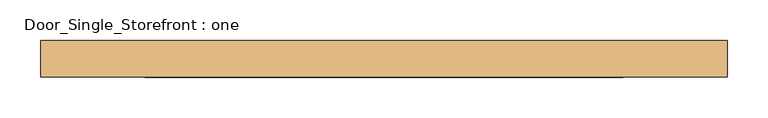
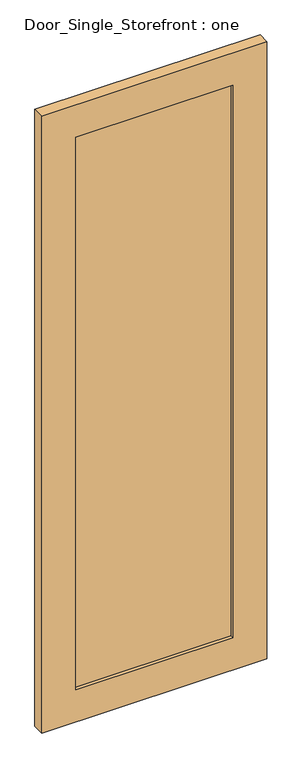
"""IFC4 building model written with IfcOpenShell, lengths in millimetres: door geometry, Door_Single_Storefront : one."""

from ifc_helpers import new_model, si_unit, frame, origin, place, context, project, spatial, polyline, outline, extrude, source, transform, mapped, element, save


def door_single_storefront_one_18792410(model_context):
    return source(origin(), model_context, "Body", "SweptSolid", [
        extrude(outline(polyline([(292.89375, -6.35), (-292.89375, -6.35), (-292.89375, 12.7), (292.89375, 12.7), (292.89375, -6.35)])), frame((0.0, 0.0, 127.0), z_axis=(0.0, 0.0, 1.0), x_axis=(1.0, 0.0, 0.0)), (0.0, 0.0, 1.0), 2178.05),
        extrude(outline(polyline([(2432.05, -419.89375), (0.0, -419.89375), (0.0, 419.89375), (2432.05, 419.89375), (2432.05, -419.89375)]), holes=[polyline([(127.0, 292.89375), (127.0, -292.89375), (2305.05, -292.89375), (2305.05, 292.89375), (127.0, 292.89375)])]), frame((0.0, -19.05, 0.0), z_axis=(0.0, 1.0, 0.0), x_axis=(0.0, 0.0, 1.0)), (0.0, 0.0, 1.0), 44.45),
    ])


if __name__ == "__main__":
    model = new_model("IFC4")
    model_context = context("Model", 3, world=origin())
    ifc_project = project(units=[si_unit("LENGTHUNIT", "METRE", prefix="MILLI")], contexts=[model_context])
    site = spatial("IfcSite", under=ifc_project)
    building = spatial("IfcBuilding", under=site)
    placement = place(None, origin())
    door_single_storefront_one_shape = door_single_storefront_one_18792410(model_context)
    element("IfcDoor", 1, ObjectType="Door_Single_Storefront : one", at=placement, inside=building, context=model_context, shape_type="MappedRepresentation", body=[
        mapped(door_single_storefront_one_shape, transform((0.0, 0.0, 0.0), x_axis=(1.0, 0.0, 0.0), y_axis=(0.0, 1.0, 0.0), z_axis=(0.0, 0.0, 1.0))),
    ])
    save(model, "model.ifc")

# Revit data of these elements
# Type "Door_Single_Storefront : one"
#   Type Mark = "27"
#   Analytic Construction = "<None>"
#   Stile_Width = 0' - 5"
#   Door_Thickness = 0' - 1 3/4"
#   Door_Offset = 0' - 1"
#   Glass_Material = SAFETY GLAZING
#   Frame_Material = INTERIOR GRADE ALUMINUM STOREFRONT W/ SAFETY GLAZING
#   Function = (empty or 0)
# Element 1 (IfcDoor, "Door_Single_Storefront : one")
#   Materials on its faces: "INTERIOR GRADE ALUMINUM STOREFRONT W/ SAFETY GLAZING", "SAFETY GLAZING"
# Materials
#   "SAFETY GLAZING": class "Glass", colour RGB 142 168 196, transparency 0.75, Description = "Soda Lime Glass", Cost = 0
#   "INTERIOR GRADE ALUMINUM STOREFRONT W/ SAFETY GLAZING": class "Metal", colour RGB 226 226 226, transparency 0, Description = "Aluminum 6061", Cost = 0
